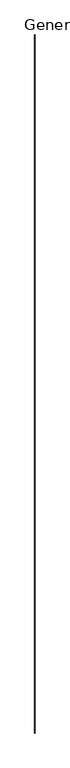
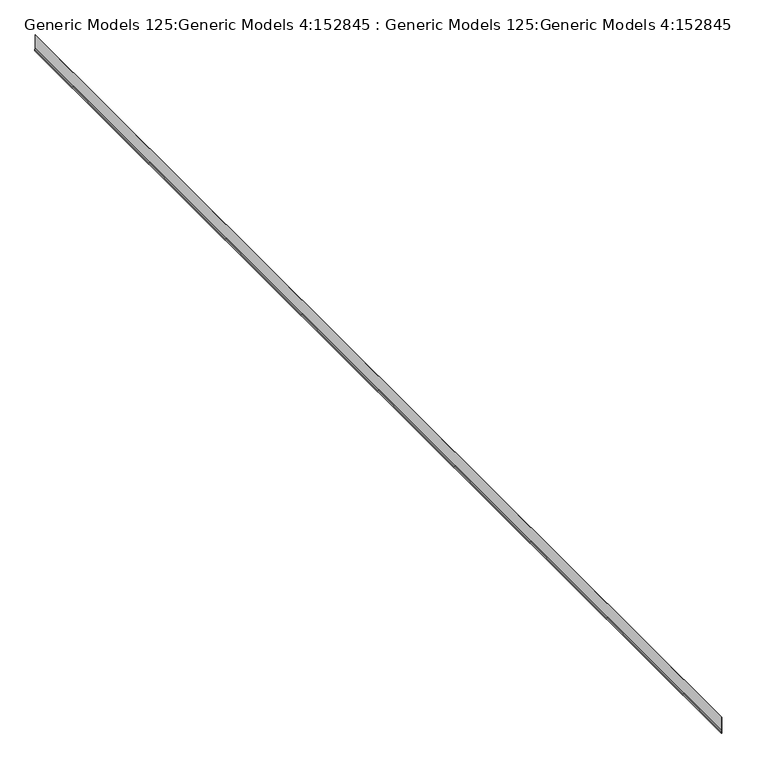
"""IFC4 building model written with IfcOpenShell, lengths in millimetres: proxy geometry, Generic Models 125:Generic Models 4:152845 : Generic Models 125:Generic Models 4:152845."""

from ifc_helpers import new_model, si_unit, frame, origin, place, context, project, spatial, polyline, outline, extrude, source, transform, mapped, element, save


def generic_models_125_generic_models_4_152845_generic_models_a513688d(model_context):
    return source(origin(), model_context, "Body", "SweptSolid", [
        extrude(outline(polyline([(2913.3927074, -6669.2783304), (2924.4864536, -6665.240537), (3067.05, -6665.240537), (3067.05, -6666.034287), (2924.6264132, -6666.034287), (2913.5326669, -6670.0720804), (2898.4789044, -6670.0720804), (2898.4789044, -6669.2783304), (2913.3927074, -6669.2783304)])), frame((0.0, -273.9974793, 0.0), z_axis=(0.0, 1.0, 0.0), x_axis=(0.0, 0.0, 1.0)), (0.0, 0.0, 1.0), 12242.8),
    ])


if __name__ == "__main__":
    model = new_model("IFC4")
    model_context = context("Model", 3, world=origin())
    ifc_project = project(units=[si_unit("LENGTHUNIT", "METRE", prefix="MILLI")], contexts=[model_context])
    site = spatial("IfcSite", under=ifc_project)
    building = spatial("IfcBuilding", under=site)
    placement = place(None, origin())
    generic_models_125_generic_models_4_152845_generic_models_shape = generic_models_125_generic_models_4_152845_generic_models_a513688d(model_context)
    element("IfcBuildingElementProxy", 1, Name="Generic Models 125:Generic Models 4:152845 : Generic Models 125:Generic Models 4:152845", ObjectType="Generic Models 125:Generic Models 4:152845 : Generic Models 125:Generic Models 4:152845", at=placement, inside=building, context=model_context, shape_type="MappedRepresentation", body=[
        mapped(generic_models_125_generic_models_4_152845_generic_models_shape, transform((0.0, 0.0, 0.0), x_axis=(1.0, 0.0, 0.0), y_axis=(0.0, 1.0, 0.0), z_axis=(0.0, 0.0, 1.0))),
    ])
    save(model, "model.ifc")

# Revit data of these elements
# Type "Generic Models 125:Generic Models 4:152845 : Generic Models 125:Generic Models 4:152845"
#   NameOverride = "Generic Models 125:Generic Models 4:152845"
#   ObjectTypeOverride = "Generic Models 125:Generic Models 4"
#   Reference = "Generic Models 4"
#   Category = "Generic Models"
#   Tag = "152845"
# Element 1 (IfcBuildingElementProxy, "Generic Models 125:Generic Models 4:152845 : Generic Models 125:Generic Models 4:152845")
#   Materials on its faces: "_(2) LAYERS NO. 30 ASTM D226 ASPHALT SATURATED ORGANIC FELT 997"
# Materials
#   "_(2) LAYERS NO. 30 ASTM D226 ASPHALT SATURATED ORGANIC FELT 997": class "Unassigned", colour RGB 67 154 161, transparency 0
